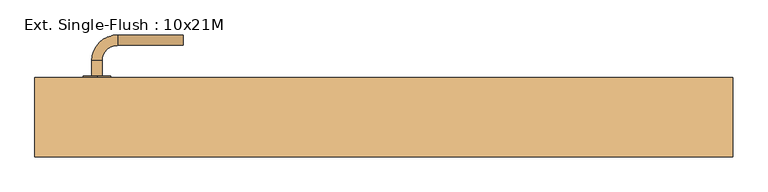
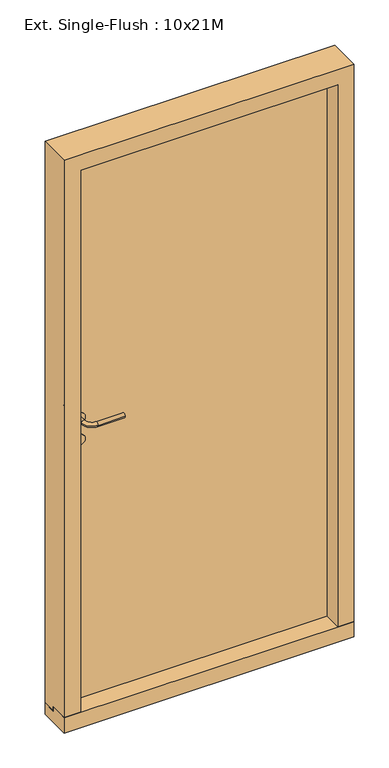
"""IFC4 building model written with IfcOpenShell, lengths in millimetres: door geometry, Ext. Single-Flush : 10x21M."""

from ifc_helpers import new_model, si_unit, point, frame, frame_2d, origin, place, context, project, spatial, polyline, circle_curve, ellipse_curve, trimmed, segment, composite_curve, outline, extrude, faceted_brep, source, transform, mapped, element, save
from ifc_brep_helpers import plane_surface, cylinder_surface, revolved_surface, advanced_brep


def ext_single_flush_10x21m_d0052ec9(model_context):
    return source(origin(), model_context, "Body", "SolidModel", [
        extrude(outline(composite_curve([segment(trimmed(circle_curve(frame_2d((1090.0, -416.0)), 20.0), [point((1070.0, -416.0))], [point((1110.0, -416.0))], False, "CARTESIAN"), True, "CONTINUOUS"), segment(trimmed(circle_curve(frame_2d((1090.0, -416.0)), 20.0), [point((1110.0, -416.0))], [point((1070.0, -416.0))], False, "CARTESIAN"), True, "CONTINUOUS")], self_intersect=False)), frame((0.0, 184.0, 0.0), z_axis=(0.0, 1.0, 0.0), x_axis=(0.0, 0.0, 1.0)), (0.0, 0.0, 1.0), 2.0),
        advanced_brep(
        [(-423.5, 186.0, 1090.0), (-408.5, 186.0, 1090.0), (-423.5, 208.5, 1090.0), (-408.5, 208.5, 1090.0), (-386.0, 231.0, 1090.0), (-386.0, 246.0, 1090.0), (-291.0, 246.0, 1090.0), (-291.0, 231.0, 1090.0)],
        [
            (0, 1, circle_curve(frame((-416.0, 186.0, 1090.0), z_axis=(0.0, -1.0, 0.0), x_axis=(1.0, 0.0, 0.0)), 7.5)),
            (1, 0, circle_curve(frame((-416.0, 186.0, 1090.0), z_axis=(0.0, -1.0, 0.0), x_axis=(1.0, 0.0, 0.0)), 7.5)),
            (0, 2),
            (2, 3, circle_curve(frame((-416.0, 208.5, 1090.0), z_axis=(0.0, -1.0, 0.0), x_axis=(1.0, 0.0, 0.0)), 7.5)),
            (3, 1),
            (3, 2, circle_curve(frame((-416.0, 208.5, 1090.0), z_axis=(0.0, -1.0, 0.0), x_axis=(1.0, 0.0, 0.0)), 7.5)),
            (4, 3, circle_curve(frame((-386.0, 208.5, 1090.0), z_axis=(0.0, 0.0, 1.0), x_axis=(-1.0, 0.0, 0.0)), 22.5)),
            (2, 5, circle_curve(frame((-386.0, 208.5, 1090.0), z_axis=(0.0, 0.0, -1.0), x_axis=(-1.0, 0.0, 0.0)), 37.5)),
            (5, 4, circle_curve(frame((-386.0, 238.5, 1090.0), z_axis=(-1.0, 0.0, 0.0), x_axis=(0.0, -1.0, 0.0)), 7.5)),
            (4, 5, circle_curve(frame((-386.0, 238.5, 1090.0), z_axis=(-1.0, 0.0, 0.0), x_axis=(0.0, -1.0, 0.0)), 7.5)),
            (5, 6),
            (6, 7, circle_curve(frame((-291.0, 238.5, 1090.0), z_axis=(-1.0, 0.0, 0.0), x_axis=(0.0, -1.0, 0.0)), 7.5)),
            (7, 4),
            (7, 6, circle_curve(frame((-291.0, 238.5, 1090.0), z_axis=(-1.0, 0.0, 0.0), x_axis=(0.0, -1.0, 0.0)), 7.5)),
        ],
        [
            plane_surface(frame((-416.0, 186.0, 1090.0), z_axis=(0.0, -1.0, 0.0), x_axis=(0.0, 0.0, -1.0))),
            cylinder_surface(frame((-416.0, 186.0, 1090.0), z_axis=(0.0, -1.0, 0.0), x_axis=(1.0, 0.0, 0.0)), 7.5),
            revolved_surface(trimmed(ellipse_curve(frame((-416.0, 208.5, 1090.0), z_axis=(0.0, -1.0, 0.0), x_axis=(1.0, 0.0, 0.0)), 7.5, 7.5), [point((-423.5, 208.5, 1090.0))], [point((-408.5, 208.5, 1090.0))], True, "CARTESIAN"), (-386.0, 208.5, 1090.0), (0.0, 0.0, -1.0)),
            revolved_surface(trimmed(ellipse_curve(frame((-416.0, 208.5, 1090.0), z_axis=(0.0, -1.0, 0.0), x_axis=(1.0, 0.0, 0.0)), 7.5, 7.5), [point((-408.5, 208.5, 1090.0))], [point((-423.5, 208.5, 1090.0))], True, "CARTESIAN"), (-386.0, 208.5, 1090.0), (0.0, 0.0, -1.0)),
            cylinder_surface(frame((-386.0, 238.5, 1090.0), z_axis=(-1.0, 0.0, 0.0), x_axis=(0.0, -1.0, 0.0)), 7.5),
            plane_surface(frame((-291.0, 238.5, 1090.0), z_axis=(1.0, 0.0, 0.0), x_axis=(0.0, 0.0, -1.0))),
        ],
        [
            (0, [[1, 2]]),
            (1, [[-1, 3, 4, 5]]),
            (1, [[-2, -5, 6, -3]]),
            (2, [[7, -4, 8, 9]]),
            (3, [[-8, -6, -7, 10]]),
            (4, [[-9, 11, 12, 13]]),
            (4, [[-10, -13, 14, -11]]),
            (5, [[-14, -12]]),
        ],
    ),
        extrude(outline(composite_curve([segment(trimmed(circle_curve(frame_2d((1010.0, -416.0)), 20.0), [point((990.0, -416.0))], [point((1030.0, -416.0))], False, "CARTESIAN"), True, "CONTINUOUS"), segment(trimmed(circle_curve(frame_2d((1010.0, -416.0)), 20.0), [point((1030.0, -416.0))], [point((990.0, -416.0))], False, "CARTESIAN"), True, "CONTINUOUS")], self_intersect=False), holes=[composite_curve([segment(trimmed(circle_curve(frame_2d((1015.0, -416.0)), 3.0), [point((1012.4019238, -417.5))], [point((1012.4019238, -414.5))], True, "CARTESIAN"), True, "CONTINUOUS"), segment(polyline([(1012.4019238, -414.5), (1000.0, -414.5), (1000.0, -417.5), (1012.4019238, -417.5)]), True, "CONTINUOUS")], self_intersect=False)]), frame((0.0, 184.0, 0.0), z_axis=(0.0, 1.0, 0.0), x_axis=(0.0, 0.0, 1.0)), (0.0, 0.0, 1.0), 2.0),
        extrude(outline(composite_curve([segment(trimmed(circle_curve(frame_2d((1090.0, -416.0)), 20.0), [point((1070.0, -416.0))], [point((1110.0, -416.0))], False, "CARTESIAN"), True, "CONTINUOUS"), segment(trimmed(circle_curve(frame_2d((1090.0, -416.0)), 20.0), [point((1110.0, -416.0))], [point((1070.0, -416.0))], False, "CARTESIAN"), True, "CONTINUOUS")], self_intersect=False)), frame((0.0, 132.0, 0.0), z_axis=(0.0, 1.0, 0.0), x_axis=(0.0, 0.0, 1.0)), (0.0, 0.0, 1.0), 2.0),
        advanced_brep(
        [(-423.5, 132.0, 1090.0), (-408.5, 132.0, 1090.0), (-408.5, 109.5, 1090.0), (-423.5, 109.5, 1090.0), (-386.0, 87.0, 1090.0), (-386.0, 72.0, 1090.0), (-291.0, 87.0, 1090.0), (-291.0, 72.0, 1090.0)],
        [
            (0, 1, circle_curve(frame((-416.0, 132.0, 1090.0), z_axis=(0.0, 1.0, 0.0), x_axis=(1.0, 0.0, 0.0)), 7.5)),
            (1, 0, circle_curve(frame((-416.0, 132.0, 1090.0), z_axis=(0.0, 1.0, 0.0), x_axis=(1.0, 0.0, 0.0)), 7.5)),
            (1, 2),
            (2, 3, circle_curve(frame((-416.0, 109.5, 1090.0), z_axis=(0.0, 1.0, 0.0), x_axis=(1.0, 0.0, 0.0)), 7.5)),
            (3, 0),
            (3, 2, circle_curve(frame((-416.0, 109.5, 1090.0), z_axis=(0.0, 1.0, 0.0), x_axis=(1.0, 0.0, 0.0)), 7.5)),
            (4, 5, circle_curve(frame((-386.0, 79.5, 1090.0), z_axis=(-1.0, 0.0, 0.0), x_axis=(0.0, 1.0, 0.0)), 7.5)),
            (5, 3, circle_curve(frame((-386.0, 109.5, 1090.0), z_axis=(0.0, 0.0, -1.0), x_axis=(-1.0, 0.0, 0.0)), 37.5)),
            (2, 4, circle_curve(frame((-386.0, 109.5, 1090.0), z_axis=(0.0, 0.0, 1.0), x_axis=(-1.0, 0.0, 0.0)), 22.5)),
            (5, 4, circle_curve(frame((-386.0, 79.5, 1090.0), z_axis=(-1.0, 0.0, 0.0), x_axis=(0.0, 1.0, 0.0)), 7.5)),
            (4, 6),
            (6, 7, circle_curve(frame((-291.0, 79.5, 1090.0), z_axis=(-1.0, 0.0, 0.0), x_axis=(0.0, 1.0, 0.0)), 7.5)),
            (7, 5),
            (7, 6, circle_curve(frame((-291.0, 79.5, 1090.0), z_axis=(-1.0, 0.0, 0.0), x_axis=(0.0, 1.0, 0.0)), 7.5)),
        ],
        [
            plane_surface(frame((-416.0, 132.0, 1090.0), z_axis=(0.0, 1.0, 0.0), x_axis=(0.0, 0.0, -1.0))),
            cylinder_surface(frame((-416.0, 132.0, 1090.0), z_axis=(0.0, 1.0, 0.0), x_axis=(1.0, 0.0, 0.0)), 7.5),
            revolved_surface(trimmed(ellipse_curve(frame((-416.0, 109.5, 1090.0), z_axis=(0.0, -1.0, 0.0), x_axis=(1.0, 0.0, 0.0)), 7.5, 7.5), [point((-423.5, 109.5, 1090.0))], [point((-408.5, 109.5, 1090.0))], True, "CARTESIAN"), (-386.0, 109.5, 1090.0), (0.0, 0.0, -1.0)),
            revolved_surface(trimmed(ellipse_curve(frame((-416.0, 109.5, 1090.0), z_axis=(0.0, -1.0, 0.0), x_axis=(1.0, 0.0, 0.0)), 7.5, 7.5), [point((-408.5, 109.5, 1090.0))], [point((-423.5, 109.5, 1090.0))], True, "CARTESIAN"), (-386.0, 109.5, 1090.0), (0.0, 0.0, -1.0)),
            cylinder_surface(frame((-386.0, 79.5, 1090.0), z_axis=(-1.0, 0.0, 0.0), x_axis=(0.0, 1.0, 0.0)), 7.5),
            plane_surface(frame((-291.0, 79.5, 1090.0), z_axis=(1.0, 0.0, 0.0), x_axis=(0.0, 0.0, -1.0))),
        ],
        [
            (0, [[1, 2]]),
            (1, [[3, 4, 5, -2]]),
            (1, [[-5, 6, -3, -1]]),
            (2, [[7, 8, -4, 9]]),
            (3, [[10, -9, -6, -8]]),
            (4, [[11, 12, 13, -7]]),
            (4, [[-13, 14, -11, -10]]),
            (5, [[-12, -14]]),
        ],
    ),
        extrude(outline(composite_curve([segment(trimmed(circle_curve(frame_2d((1010.0, -416.0)), 20.0), [point((990.0, -416.0))], [point((1030.0, -416.0))], False, "CARTESIAN"), True, "CONTINUOUS"), segment(trimmed(circle_curve(frame_2d((1010.0, -416.0)), 20.0), [point((1030.0, -416.0))], [point((990.0, -416.0))], False, "CARTESIAN"), True, "CONTINUOUS")], self_intersect=False), holes=[composite_curve([segment(trimmed(circle_curve(frame_2d((1015.0, -416.0)), 3.0), [point((1012.4019238, -417.5))], [point((1012.4019238, -414.5))], True, "CARTESIAN"), True, "CONTINUOUS"), segment(polyline([(1012.4019238, -414.5), (1000.0, -414.5), (1000.0, -417.5), (1012.4019238, -417.5)]), True, "CONTINUOUS")], self_intersect=False)]), frame((0.0, 132.0, 0.0), z_axis=(0.0, 1.0, 0.0), x_axis=(0.0, 0.0, 1.0)), (0.0, 0.0, 1.0), 2.0),
        extrude(outline(polyline([(184.0, 42.0), (184.0, 0.0), (69.0, 0.0), (69.0, 57.0), (134.0, 57.0), (134.0, 42.0), (184.0, 42.0)])), frame((-506.0, 0.0, 0.0), z_axis=(1.0, 0.0, 0.0), x_axis=(0.0, 1.0, 0.0)), (0.0, 0.0, 1.0), 1012.0),
        extrude(outline(polyline([(-464.0, 184.0), (464.0, 184.0), (464.0, 134.0), (-464.0, 134.0), (-464.0, 184.0)])), frame((0.0, 0.0, 42.0), z_axis=(0.0, 0.0, 1.0), x_axis=(1.0, 0.0, 0.0)), (0.0, 0.0, 1.0), 2028.0),
        faceted_brep([(464.0, 184.0, 2070.0), (-464.0, 184.0, 2070.0), (-464.0, 184.0, 42.0), (-506.0, 184.0, 42.0), (-506.0, 184.0, 2112.0), (506.0, 184.0, 2112.0), (506.0, 184.0, 42.0), (464.0, 184.0, 42.0), (-464.0, 134.0, 2070.0), (-464.0, 134.0, 57.0), (-464.0, 134.0, 42.0), (506.0, 134.0, 42.0), (464.0, 134.0, 42.0), (-506.0, 134.0, 42.0), (-506.0, 69.0, 2112.0), (-506.0, 134.0, 57.0), (-506.0, 69.0, 57.0), (506.0, 69.0, 2112.0), (506.0, 69.0, 57.0), (506.0, 134.0, 57.0), (464.0, 134.0, 2070.0), (464.0, 134.0, 57.0), (-449.0, 69.0, 57.0), (-449.0, 69.0, 2055.0), (449.0, 69.0, 2055.0), (449.0, 69.0, 57.0), (449.0, 134.0, 57.0), (-449.0, 134.0, 57.0), (-449.0, 134.0, 2055.0), (449.0, 134.0, 2055.0)], [[[0, 1, 2, 3, 4, 5, 6, 7]], [[1, 8, 9, 10, 2]], [[11, 12, 7, 6]], [[10, 13, 3, 2]], [[14, 4, 3, 13, 15, 16]], [[5, 17, 18, 19, 11, 6]], [[20, 0, 7, 12, 21]], [[17, 14, 16, 22, 23, 24, 25, 18]], [[21, 19, 18, 25, 26]], [[15, 9, 27, 22, 16]], [[19, 21, 12, 11]], [[9, 15, 13, 10]], [[28, 23, 22, 27]], [[24, 29, 26, 25]], [[29, 28, 27, 9, 8, 20, 21, 26]], [[5, 4, 14, 17]], [[24, 23, 28, 29]], [[1, 0, 20, 8]]]),
    ])


if __name__ == "__main__":
    model = new_model("IFC4")
    model_context = context("Model", 3, world=origin())
    ifc_project = project(units=[si_unit("LENGTHUNIT", "METRE", prefix="MILLI")], contexts=[model_context])
    site = spatial("IfcSite", under=ifc_project)
    building = spatial("IfcBuilding", under=site)
    placement = place(None, origin())
    ext_single_flush_10x21m_shape = ext_single_flush_10x21m_d0052ec9(model_context)
    element("IfcDoor", 1, ObjectType="Ext. Single-Flush : 10x21M", at=placement, inside=building, context=model_context, shape_type="MappedRepresentation", body=[
        mapped(ext_single_flush_10x21m_shape, transform((0.0, 0.0, 0.0), x_axis=(1.0, 0.0, 0.0), y_axis=(0.0, 1.0, 0.0), z_axis=(0.0, 0.0, 1.0))),
    ])
    save(model, "model.ifc")

# Revit data of these elements
# Type "Ext. Single-Flush : 10x21M"
#   Type Mark = "52"
#   Sound Rating = ""
#   Opening Side [instance default] = ""
#   Hinge Side [instance default] = ""
#   Creator Organization [instance default] = "© Danish Educational Content"
#   Creator Name [instance default] = "© Erik Falck Jørgensen"
#   Creator Build [instance default] = "2017.0801.0"
#   Analytic Construction = "<None>"
#   length#7 = -50 mm
#   length#6 = 1012 mm
#   length#5 = 120 mm
#   length#4 = 42 mm
#   length#3 = 57 mm
#   length#2a = 0 mm
#   length#2 = 0 mm
#   length#1 = 0 mm
#   Thickness = 50 mm
#   Seal Width = 12 mm
#   Rough Width = 1012 mm
#   Rough Height = 2112 mm
#   Rebate Depth = 50 mm
#   Rabbet Depth = 50 mm
#   Height = 2088 mm
#   Width = 988 mm
#   Handle From Side = 90 mm
#   Handle From Bottom = 1090 mm
#   Exterior Direction [instance default] = 0.00°
#   Case Width = 45 mm
#   Rabbet Width = 15 mm
#   Case Depth = 115 mm
#   Bottom Seal = 12 mm
#   Threshold = yes
#   Sealing = no
#   Hinging = yes
#   Wall Closure = 1
#   Function = 1
#   Panel = none
#   Handle Finish = none
#   Handle = element 507533
#   Embrasure Interior = none
#   Embrasure Exterior = none
#   Case/Transom = none
#   Assembly Code = ""
# Element 1 (IfcDoor, "Ext. Single-Flush : 10x21M")
#   Materials on its faces: "Stainless Steel, Polished", "Default Frame/Mullion (Interior/Exterior)", "Default Door Panel (Exterior/Interior)"
# Materials
#   "Stainless Steel, Polished": class "Metal", colour RGB 180 180 180, transparency 0, Description = "Rustfri stål, poleret", Cost = 0
#   "Default Frame/Mullion (Interior/Exterior)": class "Generic", colour RGB 205 205 205, transparency 0, Description = "Udefineret karm/ramme materiale", Cost = 0
#   "Default Door Panel (Exterior/Interior)": class "Generic", colour RGB 205 205 205, transparency 0, Description = "Udefineret dørplade materiale", Cost = 0
